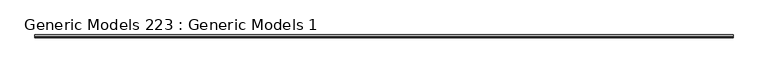
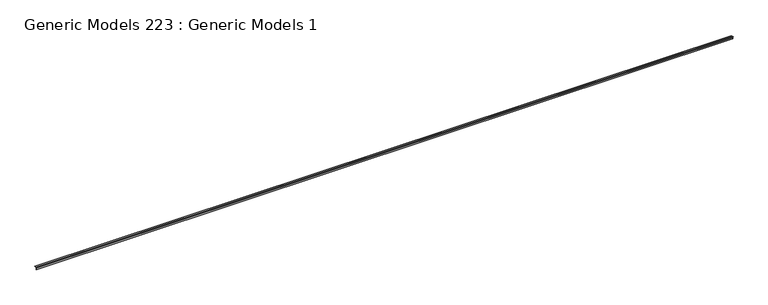
"""IFC4 building model written with IfcOpenShell, lengths in millimetres: proxy geometry, Generic Models 223 : Generic Models 1."""

import ifcopenshell
import ifcopenshell.guid

model = None  # the IFC model being written
_history = None  # IfcOwnerHistory: only IFC2X3 demands one
_inside = {}  # id of a spatial element -> (the spatial element, [elements in it])
_under = {}  # id of a project, library or spatial element -> (it, [spatial elements below it])
_declared = {}  # id of a project -> (the project, [libraries it declares])
_typed = {}  # id of a type object -> (the type object, [elements of that type])
_made_of = {}  # id of a material, layer set ... -> (it, [elements and type objects made of it])


def new_model(schema):
    """Start an empty IFC model of exactly this schema.

    Asked for "IFC4X3", IfcOpenShell would pick the latest addendum, in which some entities
    have other attributes; the version numbers below select the first issue.
    IFC2X3 requires an IfcOwnerHistory on every rooted entity: one is made here for all.
    """
    global model, _history
    if schema == "IFC4X3":
        model = ifcopenshell.file(schema_version=(4, 3, 0, 0))
    else:
        model = ifcopenshell.file(schema=schema)
    _inside.clear()
    _under.clear()
    _declared.clear()
    _typed.clear()
    _made_of.clear()
    _history = None
    if model.schema == "IFC2X3":
        org = make("IfcOrganization", Name="unknown")
        user = make(
            "IfcPersonAndOrganization",
            ThePerson=make("IfcPerson", FamilyName="unknown"),
            TheOrganization=org,
        )
        app = make(
            "IfcApplication",
            ApplicationDeveloper=org,
            Version="unknown",
            ApplicationFullName="unknown",
            ApplicationIdentifier="unknown",
        )
        _history = make(
            "IfcOwnerHistory",
            OwningUser=user,
            OwningApplication=app,
            ChangeAction="ADDED",
            CreationDate=0,
        )
    return model


def make(cls, **values):
    """One entity of the class cls with the attributes given. An attribute that is None is left unset."""
    return model.create_entity(
        cls, **{name: value for name, value in values.items() if value is not None}
    )


def rooted(cls, **values):
    """An entity with a GlobalId (a new one), such as an element, a storey or a relation."""
    return make(cls, GlobalId=ifcopenshell.guid.new(), OwnerHistory=_history, **values)


def si_unit(unit_type, name, prefix=None):
    """IfcSIUnit, for example si_unit("LENGTHUNIT", "METRE", prefix="MILLI")."""
    return make("IfcSIUnit", UnitType=unit_type, Prefix=prefix, Name=name)


def assignment(units):
    """IfcUnitAssignment: the units of a project."""
    return None if units is None else make("IfcUnitAssignment", Units=units)


def point(xyz):
    """IfcCartesianPoint."""
    return None if xyz is None else make("IfcCartesianPoint", Coordinates=xyz)


def direction(xyz):
    """IfcDirection."""
    return None if xyz is None else make("IfcDirection", DirectionRatios=xyz)


def frame(location, z_axis=None, x_axis=None):
    """IfcAxis2Placement3D, a coordinate frame: its origin and axes. An axis left out is left unset."""
    return make(
        "IfcAxis2Placement3D",
        Location=point(location),
        Axis=direction(z_axis),
        RefDirection=direction(x_axis),
    )


def frame_2d(location, x_axis=None):
    """IfcAxis2Placement2D, a coordinate frame in the plane: its origin and x axis."""
    return make(
        "IfcAxis2Placement2D", Location=point(location), RefDirection=direction(x_axis)
    )


def origin():
    """The frame at (0, 0, 0) with its axes left unset."""
    return frame((0.0, 0.0, 0.0))


def place(relative_to, where):
    """IfcLocalPlacement: puts the frame where relative to a parent placement (None: the world)."""
    return make(
        "IfcLocalPlacement", PlacementRelTo=relative_to, RelativePlacement=where
    )


def context(
    kind, dimensions, precision=None, world=None, true_north=None, identifier=None
):
    """IfcGeometricRepresentationContext, for example the 3D "Model" context."""
    return make(
        "IfcGeometricRepresentationContext",
        ContextIdentifier=identifier,
        ContextType=kind,
        CoordinateSpaceDimension=dimensions,
        Precision=precision,
        WorldCoordinateSystem=world,
        TrueNorth=true_north,
    )


def project(units=None, contexts=None):
    """IfcProject with its units and contexts."""
    return rooted(
        "IfcProject",
        Name="project",
        RepresentationContexts=contexts,
        UnitsInContext=assignment(units),
    )


def spatial(cls, under=None, at=None, **own):
    """A site, building, storey or space (cls), placed at a placement, below another one or the project."""
    s = rooted(cls, ObjectPlacement=at, **own)
    if under is not None:
        _under.setdefault(under.id(), (under, []))[1].append(s)
    return s


def polyline(points):
    """IfcPolyline through the points."""
    return make("IfcPolyline", Points=[point(p) for p in points])


def circle_curve(where, radius):
    """IfcCircle in the frame where."""
    return make("IfcCircle", Position=where, Radius=radius)


def trimmed(basis, trim1, trim2, sense, master):
    """IfcTrimmedCurve: the piece of a basis curve between two trims."""
    return make(
        "IfcTrimmedCurve",
        BasisCurve=basis,
        Trim1=trim1,
        Trim2=trim2,
        SenseAgreement=sense,
        MasterRepresentation=master,
    )


def segment(curve, same_sense, transition):
    """IfcCompositeCurveSegment."""
    return make(
        "IfcCompositeCurveSegment",
        Transition=transition,
        SameSense=same_sense,
        ParentCurve=curve,
    )


def composite_curve(segments, self_intersect=None):
    """IfcCompositeCurve: segments joined end to end."""
    return make("IfcCompositeCurve", Segments=segments, SelfIntersect=self_intersect)


def outline(outer, holes=None, kind="AREA"):
    """IfcArbitraryClosedProfileDef: a profile drawn as a closed curve; with holes, ...WithVoids."""
    if holes is None:
        return make("IfcArbitraryClosedProfileDef", ProfileType=kind, OuterCurve=outer)
    return make(
        "IfcArbitraryProfileDefWithVoids",
        ProfileType=kind,
        OuterCurve=outer,
        InnerCurves=holes,
    )


def extrude(swept, where, along, depth):
    """IfcExtrudedAreaSolid: the profile swept, set in the frame where, extruded along a direction by depth."""
    return make(
        "IfcExtrudedAreaSolid",
        SweptArea=swept,
        Position=where,
        ExtrudedDirection=direction(along),
        Depth=depth,
    )


def shape(context_of_items, identifier, shape_type, items):
    """IfcShapeRepresentation: the items that make up one representation, for example the "Body"."""
    return make(
        "IfcShapeRepresentation",
        ContextOfItems=context_of_items,
        RepresentationIdentifier=identifier,
        RepresentationType=shape_type,
        Items=items,
    )


def source(mapping_origin, context_of_items, identifier, shape_type, items):
    """IfcRepresentationMap: a shape defined once, which mapped items show again and again."""
    return make(
        "IfcRepresentationMap",
        MappingOrigin=mapping_origin,
        MappedRepresentation=shape(context_of_items, identifier, shape_type, items),
    )


def transform(
    local_origin,
    x_axis=None,
    y_axis=None,
    z_axis=None,
    scale=None,
    scale2=None,
    scale3=None,
    uniform=True,
):
    """IfcCartesianTransformationOperator3D, or its non-uniform kind. x_axis, y_axis, z_axis: its Axis1, 2, 3."""
    if uniform:
        return make(
            "IfcCartesianTransformationOperator3D",
            Axis1=direction(x_axis),
            Axis2=direction(y_axis),
            LocalOrigin=point(local_origin),
            Scale=scale,
            Axis3=direction(z_axis),
        )
    return make(
        "IfcCartesianTransformationOperator3DnonUniform",
        Axis1=direction(x_axis),
        Axis2=direction(y_axis),
        LocalOrigin=point(local_origin),
        Scale=scale,
        Axis3=direction(z_axis),
        Scale2=scale2,
        Scale3=scale3,
    )


def mapped(mapping_source, mapping_target):
    """IfcMappedItem: shows the shape of a source again, moved by a transform."""
    return make(
        "IfcMappedItem", MappingSource=mapping_source, MappingTarget=mapping_target
    )


def made_of(thing, what):
    """Note that an element or type object is made of a material, layer set ...; save() writes the relation."""
    if what is not None:
        _made_of.setdefault(what.id(), (what, []))[1].append(thing)
    return thing


def element(
    cls,
    number,
    at=None,
    inside=None,
    cuts=None,
    type_object=None,
    material=None,
    context=None,
    identifier="Body",
    shape_type=None,
    held_by="IfcProductDefinitionShape",
    body=None,
    shapes=None,
    **own,
):
    """One element of the class cls, such as IfcWall. Its Tag is "e" and its number.

    at: its placement. inside: the storey or other place that contains it. cuts: it is an
    opening in that element (IfcRelVoidsElement). A single representation is given by context,
    identifier, shape_type and body (its items); several are given by shapes. held_by: the class
    of the entity that holds the representations. save() writes the other relations.
    """
    e = rooted(cls, Tag="e%d" % number, ObjectPlacement=at, **own)
    if body is not None:
        shapes = [shape(context, identifier, shape_type, body)]
    if shapes is not None:
        e.Representation = make(held_by, Representations=shapes)
    if inside is not None:
        _inside.setdefault(inside.id(), (inside, []))[1].append(e)
    if cuts is not None:
        rooted(
            "IfcRelVoidsElement", RelatingBuildingElement=cuts, RelatedOpeningElement=e
        )
    if type_object is not None:
        _typed.setdefault(type_object.id(), (type_object, []))[1].append(e)
    return made_of(e, material)


def aggregate(whole, parts):
    """IfcRelAggregates: a whole, such as a stair, and the parts it consists of."""
    return rooted("IfcRelAggregates", RelatingObject=whole, RelatedObjects=parts)


def save(model, path):
    """Write the relations noted so far, then the file.

    IfcRelAggregates (storeys below a building ...), IfcRelContainedInSpatialStructure (elements
    in a storey), IfcRelDefinesByType, IfcRelAssociatesMaterial and IfcRelDeclares: one each for
    every whole, place, type object, material and project.
    """
    for whole, parts in _under.values():
        aggregate(whole, parts)
    for where, things in _inside.values():
        rooted(
            "IfcRelContainedInSpatialStructure",
            RelatedElements=things,
            RelatingStructure=where,
        )
    for kind, things in _typed.values():
        rooted("IfcRelDefinesByType", RelatedObjects=things, RelatingType=kind)
    for what, things in _made_of.values():
        rooted("IfcRelAssociatesMaterial", RelatedObjects=things, RelatingMaterial=what)
    for by, libraries in _declared.values():
        rooted("IfcRelDeclares", RelatingContext=by, RelatedDefinitions=libraries)
    model.write(path)


def generic_models_223_generic_models_1_2f6ac014(model_context):
    return source(origin(), model_context, "Body", "SweptSolid", [
        extrude(outline(composite_curve([segment(polyline([(-29401.8740187, 127166.5926156), (-29363.8485041, 127147.066), (-29325.7485041, 127147.066), (-29325.7485041, 127145.796), (-29364.1555279, 127145.796), (-29402.9086261, 127165.6962396), (-29383.0083865, 127126.9431414), (-29383.0083865, 127088.5361176), (-29384.2783865, 127088.5361176), (-29384.2783865, 127126.6361176), (-29403.8050021, 127164.6616323)]), True, "CONTINUOUS"), segment(trimmed(circle_curve(frame_2d((-29402.5291738, 127165.3167873)), 1.4342127), [point((-29403.8050021, 127164.6616323))], [point((-29401.8740187, 127166.5926156))], False, "CARTESIAN"), True, "CONTINUOUS")], self_intersect=False)), frame((-20998.9733045, 0.0, 0.0), z_axis=(1.0, 0.0, 0.0), x_axis=(0.0, 1.0, 0.0)), (0.0, 0.0, 1.0), 19050.0),
    ])


if __name__ == "__main__":
    model = new_model("IFC4")
    model_context = context("Model", 3, world=origin())
    ifc_project = project(units=[si_unit("LENGTHUNIT", "METRE", prefix="MILLI")], contexts=[model_context])
    site = spatial("IfcSite", under=ifc_project)
    building = spatial("IfcBuilding", under=site)
    placement = place(None, origin())
    generic_models_223_generic_models_1_shape = generic_models_223_generic_models_1_2f6ac014(model_context)
    element("IfcBuildingElementProxy", 1, Name="Generic Models 223 : Generic Models 1", ObjectType="Generic Models 223 : Generic Models 1", at=placement, inside=building, context=model_context, shape_type="MappedRepresentation", body=[
        mapped(generic_models_223_generic_models_1_shape, transform((0.0, 0.0, 0.0), x_axis=(1.0, 0.0, 0.0), y_axis=(0.0, 1.0, 0.0), z_axis=(0.0, 0.0, 1.0))),
    ])
    save(model, "model.ifc")

# Revit data of these elements
# Element 1 (IfcBuildingElementProxy, "Generic Models 223 : Generic Models 1")
#   Materials on its faces: "_CONTINIOUS 16 GA. COPPER CORNER BEAD"
# Materials
#   "_CONTINIOUS 16 GA. COPPER CORNER BEAD": class "Generic", colour RGB 253 192 103, transparency 0, Cost = 0
